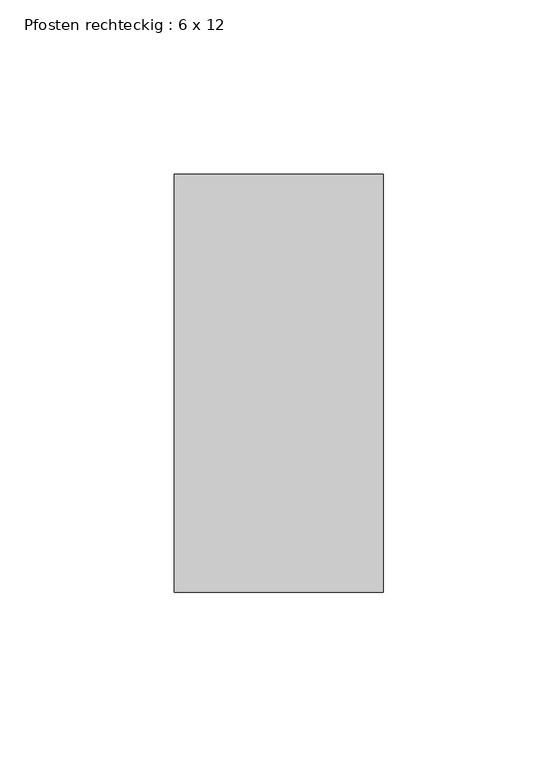
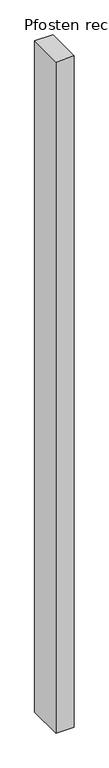
"""IFC4 building model written with IfcOpenShell, lengths in millimetres: member geometry, Pfosten rechteckig : 6 x 12."""

from ifc_helpers import new_model, si_unit, frame, origin, place, context, project, spatial, polyline, outline, extrude, source, transform, mapped, element, save


def pfosten_rechteckig_6_x_12_7e254c8a(model_context):
    return source(origin(), model_context, "Body", "SweptSolid", [
        extrude(outline(polyline([(0.0, 60.0), (0.0, -60.0), (-60.0, -60.0), (-60.0, 60.0), (0.0, 60.0)])), frame((0.0, 0.0, -2320.0), z_axis=(0.0, 0.0, 1.0), x_axis=(1.0, 0.0, 0.0)), (0.0, 0.0, 1.0), 2320.0),
    ])


if __name__ == "__main__":
    model = new_model("IFC4")
    model_context = context("Model", 3, world=origin())
    ifc_project = project(units=[si_unit("LENGTHUNIT", "METRE", prefix="MILLI")], contexts=[model_context])
    site = spatial("IfcSite", under=ifc_project)
    building = spatial("IfcBuilding", under=site)
    placement = place(None, origin())
    pfosten_rechteckig_6_x_12_shape = pfosten_rechteckig_6_x_12_7e254c8a(model_context)
    element("IfcMember", 1, ObjectType="Pfosten rechteckig : 6 x 12", at=placement, inside=building, context=model_context, shape_type="MappedRepresentation", body=[
        mapped(pfosten_rechteckig_6_x_12_shape, transform((0.0, 0.0, 0.0), x_axis=(1.0, 0.0, 0.0), y_axis=(0.0, 1.0, 0.0), z_axis=(0.0, 0.0, 1.0))),
    ])
    save(model, "model.ifc")

# Revit data of these elements
# Type "Pfosten rechteckig : 6 x 12"
#   built-in parameter 1007304 = 0.393701 (stored number, unit not read)
#   built-in parameter 1007301 = 0.0984252 (stored number, unit not read)
#   built-in parameter 1007300 = 0.0984252 (stored number, unit not read)
# Element 1 (IfcMember, "Pfosten rechteckig : 6 x 12")
#   Materials on its faces: "Metall - verzinkt"
# Materials
#   "Metall - verzinkt": class "Allgemeines", colour RGB 200 200 200, transparency 0, Cost = 0
